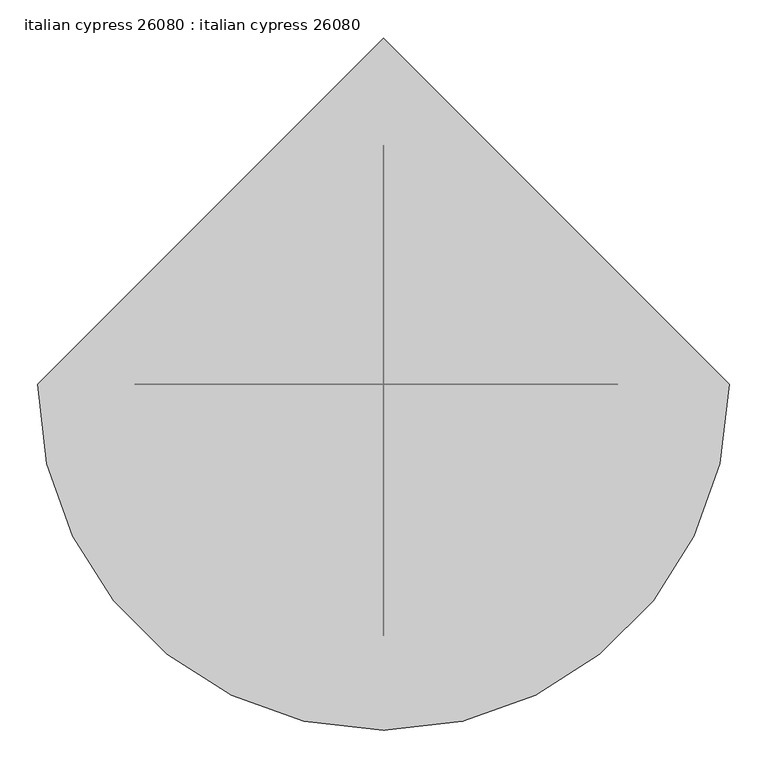
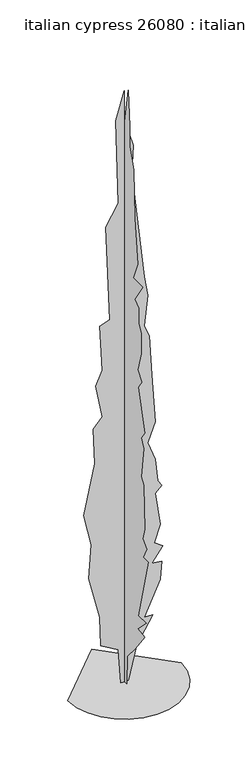
"""IFC4 building model written with IfcOpenShell, lengths in millimetres: proxy geometry, italian cypress 26080 : italian cypress 26080."""

from ifc_helpers import new_model, si_unit, origin, place, context, project, spatial, triangles, source, transform, mapped, element, save


def italian_cypress_26080_italian_cypress_26080_3042d0aa(model_context):
    return source(origin(), model_context, "Body", "Tessellation", [
        triangles([(-29.5869341, 1.3e-06, 0.1194313), (-49.5769884, -1.53e-05, 292.3971778), (-189.5068557, -1.39e-05, 372.3589213), (-199.501758, -2.84e-05, 622.2339672), (-289.4558421, -4.59e-05, 982.0528473), (-269.4660557, -6.34e-05, 1261.9126545), (-329.4354512, -7.69e-05, 1531.7774323), (-239.4816032, -0.0001053, 1941.5708782), (-249.4767599, -0.0001227, 2241.4229244), (-179.5116991, -0.0001305, 2321.3821426), (-229.486701, -0.000145, 2601.2391884), (-179.5116991, -0.0001543, 2721.1780884), (-199.501758, -0.0001761, 3100.9842659), (-119.5417949, -0.0001814, 3130.9815628), (-149.526747, -0.0002277, 3930.573745), (-49.5767341, -0.0002422, 4100.4997101), (-69.5667884, -0.0002837, 4810.1247093), (0.3982034, -0.0003004, 5040.0202698), (0.3981933, -0.0002861, 4800.1427605), (70.3630788, -0.0002743, 4550.2574318), (60.3681766, -0.0002602, 4320.3874512), (160.3179397, -0.0002097, 3400.8313705), (190.3028827, -0.0002009, 3230.9306946), (160.3179397, -0.0001847, 2981.0453659), (200.2977849, -0.0001805, 2881.0965248), (220.2878438, -0.0001611, 2541.2698837), (250.2727869, -0.000138, 2131.4764378), (190.3028827, -0.0001258, 1971.5581467), (250.2727869, -0.0001189, 1811.6370941), (270.2636088, -0.0001085, 1621.7315346), (300.2483156, -0.0001068, 1571.7569687), (250.2727869, -0.0001016, 1521.7825481), (290.2534133, -8.67e-05, 1241.9227409), (240.2779027, -7.62e-05, 1101.9916746), (310.2431997, -7.63e-05, 1052.0171814), (220.2878438, -6.52e-05, 932.0783541), (300.2483156, -6.81e-05, 922.08347), (290.2534133, -5.87e-05, 772.1574469), (160.3179397, -3.64e-05, 492.2977123), (230.2827461, -3.94e-05, 492.2977123), (100.347772, -2.12e-05, 282.4022756), (30.3829701, -1.3e-06, 0.0599298), (2.7e-06, 26.9145999, 3.61e-05), (9.8e-06, 16.9195239, 242.4231751), (1.41e-05, 96.8794064, 262.412471), (2.63e-05, 206.8243124, 502.2925964), (4.24e-05, 316.7684555, 832.1268242), (4.2e-05, 236.8092736, 902.0937017), (4.85e-05, 246.8041759, 1111.9865587), (5.8e-05, 276.7888646, 1441.8233299), (6.33e-05, 266.7939623, 1571.7569687), (6.23e-05, 216.8192147, 1671.7059551), (7.15e-05, 276.7888646, 1891.5963123), (7.8e-05, 196.8291558, 2191.4458878), (7.92e-05, 176.8393694, 2311.3872585), (8.8e-05, 226.814117, 2461.3108109), (8.96e-05, 166.8442128, 2701.1883202), (9.57e-05, 176.8391151, 2831.1347488), (9.7e-05, 136.8592607, 2971.0634171), (0.0001065, 156.8493105, 3240.9129341), (0.0001061, 86.8842497, 3370.8593628), (0.0001161, 126.8643584, 3560.749807), (0.0001208, 76.8893565, 3860.6219101), (0.0001291, 36.9092456, 4160.4690147), (0.0001382, 66.8941999, 4410.3287636), (0.000139, 26.9143478, 4540.2751923), (0.0001451, -3.0706568, 4780.1527016), (0.0001529, -53.045613, 5079.9998062), (0.000142, -73.0356673, 4780.1527016), (0.0001377, -73.0356673, 4610.2267365), (0.0001312, -133.0055715, 4450.3083), (0.0001159, -143.0004738, 4040.5301147), (0.0001043, -182.9803282, 3670.7061768), (0.0001034, -123.0104149, 3520.7699799), (9.77e-05, -252.945389, 3520.7699799), (9.51e-05, -143.0004738, 3350.8695946), (9.39e-05, -202.9703689, 3310.8897675), (8.82e-05, -202.9703689, 3180.9433388), (8.38e-05, -232.9553301, 3110.9917946), (7.95e-05, -232.9553301, 2941.0658295), (7.74e-05, -182.9803282, 2771.1651535), (7.17e-05, -242.9502324, 2701.1883202), (7.39e-05, -192.9754848, 2631.236776), (5.82e-05, -282.9305863, 2291.397345), (5.74e-05, -232.9553301, 2221.4331562), (5.57e-05, -272.9356841, 2151.466206), (4.92e-05, -232.9553301, 1891.5963123), (4.52e-05, -272.9356841, 1841.6218918), (3.49e-05, -282.9305863, 1471.8079823), (3.18e-05, -252.9451346, 1371.856525), (2.7e-05, -312.915275, 1321.8819592), (2.79e-05, -262.9407818, 1221.9329727), (2.49e-05, -332.9050796, 1221.9329727), (1.36e-05, -192.9752305, 682.2033445), (8.8e-06, -302.9203909, 682.2033445), (1.19e-05, -182.9803282, 562.2620101), (7.1e-06, -282.9305863, 552.2670897), (8e-06, -152.995367, 372.3589213), (7.2e-06, -43.0504564, 242.4231751), (1e-07, -33.0553043, 3.25e-05), (-457.8197296, 0.0, 5.45e-05), (-445.716653, -104.9022542, 4.77e-05), (-411.2488441, -201.2383525, 4.05e-05), (-357.1696959, -286.2478257, 3.3e-05), (-286.2478257, -357.1722393, 2.57e-05), (-201.2380982, -411.2463006, 1.88e-05), (-104.9022542, -445.716653, 1.25e-05), (2.2e-05, -457.8222731, 7.2e-06), (104.9022542, -445.716653, 3.3e-06), (201.2383525, -411.2488441, 1.2e-06), (286.2478257, -357.1696959, 7e-07), (357.1722393, -286.2478257, 1.8e-06), (411.2463006, -201.2380982, 4.5e-06), (445.716653, -104.9022542, 8.7e-06), (457.8197296, 4e-05, 1.45e-05), (-5.93e-05, 457.8222731, 6.18e-05)], [[17, 18, 19], [39, 40, 41], [16, 17, 19], [16, 19, 20], [16, 20, 21], [16, 21, 22], [15, 16, 22], [14, 15, 22], [14, 22, 23], [14, 23, 24], [34, 35, 36], [36, 37, 38], [42, 1, 2], [41, 42, 2], [39, 41, 2], [30, 31, 32], [39, 2, 3], [39, 3, 4], [38, 39, 4], [36, 38, 4], [36, 4, 5], [34, 36, 5], [34, 5, 6], [33, 34, 6], [32, 33, 6], [32, 6, 7], [32, 7, 8], [30, 32, 8], [29, 30, 8], [28, 29, 8], [28, 8, 9], [27, 28, 9], [27, 9, 10], [26, 27, 10], [26, 10, 11], [26, 11, 12], [25, 26, 12], [25, 12, 13], [24, 25, 13], [14, 24, 13], [67, 68, 69], [94, 95, 96], [74, 75, 76], [96, 97, 98], [92, 93, 94], [100, 43, 44], [99, 100, 44], [67, 69, 70], [66, 67, 70], [66, 70, 71], [65, 66, 71], [65, 71, 72], [64, 65, 72], [63, 64, 72], [63, 72, 73], [62, 63, 73], [62, 73, 74], [61, 62, 74], [61, 74, 76], [90, 91, 92], [81, 82, 83], [46, 47, 48], [60, 61, 76], [59, 60, 76], [59, 76, 77], [59, 77, 78], [59, 78, 79], [59, 79, 80], [59, 80, 81], [58, 59, 81], [57, 58, 81], [57, 81, 83], [56, 57, 83], [56, 83, 84], [55, 56, 84], [55, 84, 85], [54, 55, 85], [53, 54, 85], [53, 85, 86], [53, 86, 87], [52, 53, 87], [52, 87, 88], [52, 88, 89], [51, 52, 89], [51, 89, 90], [50, 51, 90], [49, 50, 90], [49, 90, 92], [49, 92, 94], [48, 49, 94], [46, 48, 94], [46, 94, 96], [46, 96, 98], [45, 46, 98], [45, 98, 99], [44, 45, 99], [115, 116, 101], [114, 115, 101], [114, 101, 102], [113, 114, 102], [113, 102, 103], [113, 103, 104], [112, 113, 104], [111, 112, 104], [111, 104, 105], [111, 105, 106], [111, 106, 107], [111, 107, 108], [111, 108, 109], [111, 109, 110]], closed=False),
    ])


if __name__ == "__main__":
    model = new_model("IFC4")
    model_context = context("Model", 3, world=origin())
    ifc_project = project(units=[si_unit("LENGTHUNIT", "METRE", prefix="MILLI")], contexts=[model_context])
    site = spatial("IfcSite", under=ifc_project)
    building = spatial("IfcBuilding", under=site)
    placement = place(None, origin())
    italian_cypress_26080_italian_cypress_26080_shape = italian_cypress_26080_italian_cypress_26080_3042d0aa(model_context)
    element("IfcBuildingElementProxy", 1, Name="italian cypress 26080 : italian cypress 26080", ObjectType="italian cypress 26080 : italian cypress 26080", at=placement, inside=building, context=model_context, shape_type="MappedRepresentation", body=[
        mapped(italian_cypress_26080_italian_cypress_26080_shape, transform((0.0, 0.0, 0.0), x_axis=(1.0, 0.0, 0.0), y_axis=(0.0, 1.0, 0.0), z_axis=(0.0, 0.0, 1.0))),
    ])
    save(model, "model.ifc")

# Revit data of these elements
# Type "italian cypress 26080 : italian cypress 26080"
#   built-in parameter 1005195 = "RPC-16-FWM7-6P00-C8X0-C000-ST1L-LVER-AU"
#   Height = 0
